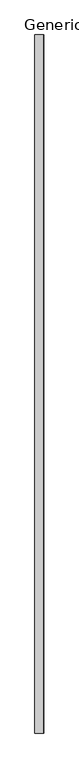
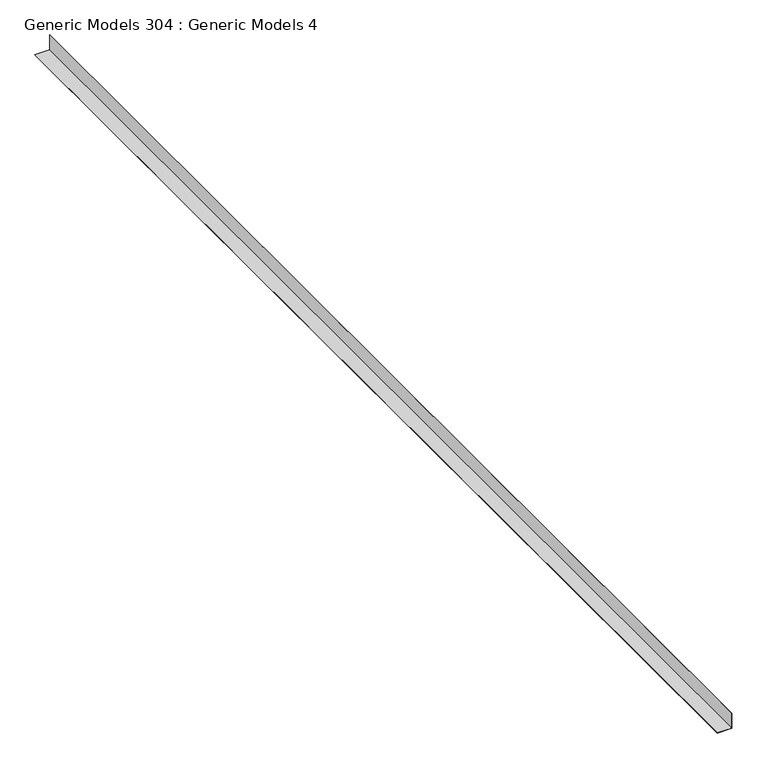
"""IFC4 building model written with IfcOpenShell, lengths in millimetres: proxy geometry, Generic Models 304 : Generic Models 4."""

from ifc_helpers import new_model, si_unit, frame, origin, place, context, project, spatial, polyline, outline, extrude, source, transform, mapped, element, save


def generic_models_304_generic_models_4_800efd7f(model_context):
    return source(origin(), model_context, "Body", "SweptSolid", [
        extrude(outline(polyline([(129227.0085, 4942.5173808), (129227.0085, 4843.1531101), (129226.21475, 4843.1531101), (129226.21475, 4943.3111308), (129333.7747679, 4943.3111308), (129333.7747679, 4942.5173808), (129227.0085, 4942.5173808)])), frame((0.0, -2626.9952162, 0.0), z_axis=(0.0, 1.0, 0.0), x_axis=(0.0, 0.0, 1.0)), (0.0, 0.0, 1.0), 7999.1330657),
    ])


if __name__ == "__main__":
    model = new_model("IFC4")
    model_context = context("Model", 3, world=origin())
    ifc_project = project(units=[si_unit("LENGTHUNIT", "METRE", prefix="MILLI")], contexts=[model_context])
    site = spatial("IfcSite", under=ifc_project)
    building = spatial("IfcBuilding", under=site)
    placement = place(None, origin())
    generic_models_304_generic_models_4_shape = generic_models_304_generic_models_4_800efd7f(model_context)
    element("IfcBuildingElementProxy", 1, Name="Generic Models 304 : Generic Models 4", ObjectType="Generic Models 304 : Generic Models 4", at=placement, inside=building, context=model_context, shape_type="MappedRepresentation", body=[
        mapped(generic_models_304_generic_models_4_shape, transform((0.0, 0.0, 0.0), x_axis=(1.0, 0.0, 0.0), y_axis=(0.0, 1.0, 0.0), z_axis=(0.0, 0.0, 1.0))),
    ])
    save(model, "model.ifc")

# Revit data of these elements
# Element 1 (IfcBuildingElementProxy, "Generic Models 304 : Generic Models 4")
#   Materials on its faces: "_SELF ADHERED MEMBRANE"
# Materials
#   "_SELF ADHERED MEMBRANE": class "Generic", colour RGB 253 192 103, transparency 0, Cost = 0
